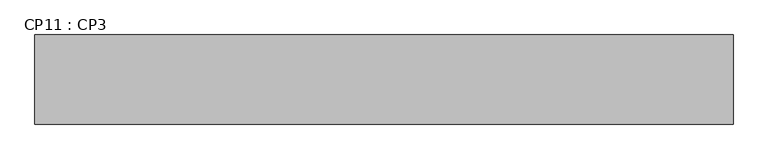
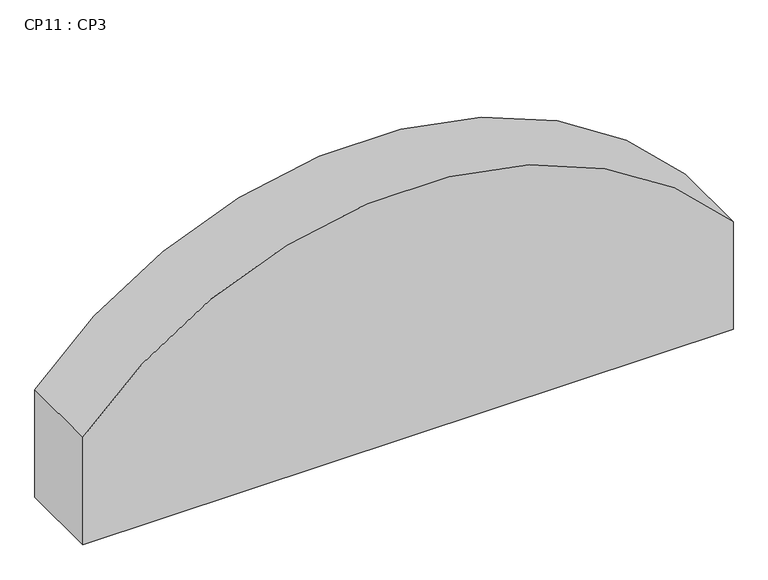
"""IFC4 building model written with IfcOpenShell, lengths in millimetres: beam geometry, CP11 : CP3."""

import ifcopenshell
import ifcopenshell.guid

model = None  # the IFC model being written
_history = None  # IfcOwnerHistory: only IFC2X3 demands one
_inside = {}  # id of a spatial element -> (the spatial element, [elements in it])
_under = {}  # id of a project, library or spatial element -> (it, [spatial elements below it])
_declared = {}  # id of a project -> (the project, [libraries it declares])
_typed = {}  # id of a type object -> (the type object, [elements of that type])
_made_of = {}  # id of a material, layer set ... -> (it, [elements and type objects made of it])


def new_model(schema):
    """Start an empty IFC model of exactly this schema.

    Asked for "IFC4X3", IfcOpenShell would pick the latest addendum, in which some entities
    have other attributes; the version numbers below select the first issue.
    IFC2X3 requires an IfcOwnerHistory on every rooted entity: one is made here for all.
    """
    global model, _history
    if schema == "IFC4X3":
        model = ifcopenshell.file(schema_version=(4, 3, 0, 0))
    else:
        model = ifcopenshell.file(schema=schema)
    _inside.clear()
    _under.clear()
    _declared.clear()
    _typed.clear()
    _made_of.clear()
    _history = None
    if model.schema == "IFC2X3":
        org = make("IfcOrganization", Name="unknown")
        user = make(
            "IfcPersonAndOrganization",
            ThePerson=make("IfcPerson", FamilyName="unknown"),
            TheOrganization=org,
        )
        app = make(
            "IfcApplication",
            ApplicationDeveloper=org,
            Version="unknown",
            ApplicationFullName="unknown",
            ApplicationIdentifier="unknown",
        )
        _history = make(
            "IfcOwnerHistory",
            OwningUser=user,
            OwningApplication=app,
            ChangeAction="ADDED",
            CreationDate=0,
        )
    return model


def make(cls, **values):
    """One entity of the class cls with the attributes given. An attribute that is None is left unset."""
    return model.create_entity(
        cls, **{name: value for name, value in values.items() if value is not None}
    )


def rooted(cls, **values):
    """An entity with a GlobalId (a new one), such as an element, a storey or a relation."""
    return make(cls, GlobalId=ifcopenshell.guid.new(), OwnerHistory=_history, **values)


def si_unit(unit_type, name, prefix=None):
    """IfcSIUnit, for example si_unit("LENGTHUNIT", "METRE", prefix="MILLI")."""
    return make("IfcSIUnit", UnitType=unit_type, Prefix=prefix, Name=name)


def assignment(units):
    """IfcUnitAssignment: the units of a project."""
    return None if units is None else make("IfcUnitAssignment", Units=units)


def point(xyz):
    """IfcCartesianPoint."""
    return None if xyz is None else make("IfcCartesianPoint", Coordinates=xyz)


def direction(xyz):
    """IfcDirection."""
    return None if xyz is None else make("IfcDirection", DirectionRatios=xyz)


def frame(location, z_axis=None, x_axis=None):
    """IfcAxis2Placement3D, a coordinate frame: its origin and axes. An axis left out is left unset."""
    return make(
        "IfcAxis2Placement3D",
        Location=point(location),
        Axis=direction(z_axis),
        RefDirection=direction(x_axis),
    )


def origin():
    """The frame at (0, 0, 0) with its axes left unset."""
    return frame((0.0, 0.0, 0.0))


def place(relative_to, where):
    """IfcLocalPlacement: puts the frame where relative to a parent placement (None: the world)."""
    return make(
        "IfcLocalPlacement", PlacementRelTo=relative_to, RelativePlacement=where
    )


def context(
    kind, dimensions, precision=None, world=None, true_north=None, identifier=None
):
    """IfcGeometricRepresentationContext, for example the 3D "Model" context."""
    return make(
        "IfcGeometricRepresentationContext",
        ContextIdentifier=identifier,
        ContextType=kind,
        CoordinateSpaceDimension=dimensions,
        Precision=precision,
        WorldCoordinateSystem=world,
        TrueNorth=true_north,
    )


def project(units=None, contexts=None):
    """IfcProject with its units and contexts."""
    return rooted(
        "IfcProject",
        Name="project",
        RepresentationContexts=contexts,
        UnitsInContext=assignment(units),
    )


def spatial(cls, under=None, at=None, **own):
    """A site, building, storey or space (cls), placed at a placement, below another one or the project."""
    s = rooted(cls, ObjectPlacement=at, **own)
    if under is not None:
        _under.setdefault(under.id(), (under, []))[1].append(s)
    return s


def circle_curve(where, radius):
    """IfcCircle in the frame where."""
    return make("IfcCircle", Position=where, Radius=radius)


def shape(context_of_items, identifier, shape_type, items):
    """IfcShapeRepresentation: the items that make up one representation, for example the "Body"."""
    return make(
        "IfcShapeRepresentation",
        ContextOfItems=context_of_items,
        RepresentationIdentifier=identifier,
        RepresentationType=shape_type,
        Items=items,
    )


def source(mapping_origin, context_of_items, identifier, shape_type, items):
    """IfcRepresentationMap: a shape defined once, which mapped items show again and again."""
    return make(
        "IfcRepresentationMap",
        MappingOrigin=mapping_origin,
        MappedRepresentation=shape(context_of_items, identifier, shape_type, items),
    )


def transform(
    local_origin,
    x_axis=None,
    y_axis=None,
    z_axis=None,
    scale=None,
    scale2=None,
    scale3=None,
    uniform=True,
):
    """IfcCartesianTransformationOperator3D, or its non-uniform kind. x_axis, y_axis, z_axis: its Axis1, 2, 3."""
    if uniform:
        return make(
            "IfcCartesianTransformationOperator3D",
            Axis1=direction(x_axis),
            Axis2=direction(y_axis),
            LocalOrigin=point(local_origin),
            Scale=scale,
            Axis3=direction(z_axis),
        )
    return make(
        "IfcCartesianTransformationOperator3DnonUniform",
        Axis1=direction(x_axis),
        Axis2=direction(y_axis),
        LocalOrigin=point(local_origin),
        Scale=scale,
        Axis3=direction(z_axis),
        Scale2=scale2,
        Scale3=scale3,
    )


def mapped(mapping_source, mapping_target):
    """IfcMappedItem: shows the shape of a source again, moved by a transform."""
    return make(
        "IfcMappedItem", MappingSource=mapping_source, MappingTarget=mapping_target
    )


def made_of(thing, what):
    """Note that an element or type object is made of a material, layer set ...; save() writes the relation."""
    if what is not None:
        _made_of.setdefault(what.id(), (what, []))[1].append(thing)
    return thing


def element(
    cls,
    number,
    at=None,
    inside=None,
    cuts=None,
    type_object=None,
    material=None,
    context=None,
    identifier="Body",
    shape_type=None,
    held_by="IfcProductDefinitionShape",
    body=None,
    shapes=None,
    **own,
):
    """One element of the class cls, such as IfcWall. Its Tag is "e" and its number.

    at: its placement. inside: the storey or other place that contains it. cuts: it is an
    opening in that element (IfcRelVoidsElement). A single representation is given by context,
    identifier, shape_type and body (its items); several are given by shapes. held_by: the class
    of the entity that holds the representations. save() writes the other relations.
    """
    e = rooted(cls, Tag="e%d" % number, ObjectPlacement=at, **own)
    if body is not None:
        shapes = [shape(context, identifier, shape_type, body)]
    if shapes is not None:
        e.Representation = make(held_by, Representations=shapes)
    if inside is not None:
        _inside.setdefault(inside.id(), (inside, []))[1].append(e)
    if cuts is not None:
        rooted(
            "IfcRelVoidsElement", RelatingBuildingElement=cuts, RelatedOpeningElement=e
        )
    if type_object is not None:
        _typed.setdefault(type_object.id(), (type_object, []))[1].append(e)
    return made_of(e, material)


def aggregate(whole, parts):
    """IfcRelAggregates: a whole, such as a stair, and the parts it consists of."""
    return rooted("IfcRelAggregates", RelatingObject=whole, RelatedObjects=parts)


def save(model, path):
    """Write the relations noted so far, then the file.

    IfcRelAggregates (storeys below a building ...), IfcRelContainedInSpatialStructure (elements
    in a storey), IfcRelDefinesByType, IfcRelAssociatesMaterial and IfcRelDeclares: one each for
    every whole, place, type object, material and project.
    """
    for whole, parts in _under.values():
        aggregate(whole, parts)
    for where, things in _inside.values():
        rooted(
            "IfcRelContainedInSpatialStructure",
            RelatedElements=things,
            RelatingStructure=where,
        )
    for kind, things in _typed.values():
        rooted("IfcRelDefinesByType", RelatedObjects=things, RelatingType=kind)
    for what, things in _made_of.values():
        rooted("IfcRelAssociatesMaterial", RelatedObjects=things, RelatingMaterial=what)
    for by, libraries in _declared.values():
        rooted("IfcRelDeclares", RelatingContext=by, RelatedDefinitions=libraries)
    model.write(path)


def plane_surface(at):
    """IfcPlane: the flat surface through the origin of the frame at, square to its z axis."""
    return make("IfcPlane", Position=at)


def cylinder_surface(at, radius):
    """IfcCylindricalSurface: all points at the distance radius from the z axis of the frame at."""
    return make("IfcCylindricalSurface", Position=at, Radius=radius)


def advanced_brep(points, edges, surfaces, faces):
    """IfcAdvancedBrep: a solid bounded by faces that lie on surfaces and meet in shared edges.

    An edge is (start, end): straight between two places in points (the first is 0);
    or (start, end, curve); or (start, end, curve, False) where it runs against its curve.
    A face is (place in surfaces, loops), or (place, loops, False) where it looks against
    its surface's normal. A loop lists edges by number (the first is 1), with a minus sign
    where the edge is run from its end to its start. The first loop is the outer one.
    """
    corners = [point(p) for p in points]
    vertices = [make("IfcVertexPoint", VertexGeometry=c) for c in corners]
    made = []
    for start, end, *more in edges:
        made.append(
            make(
                "IfcEdgeCurve",
                EdgeStart=vertices[start],
                EdgeEnd=vertices[end],
                EdgeGeometry=more[0] if more else make("IfcPolyline", Points=[corners[start], corners[end]]),
                SameSense=more[1] if len(more) > 1 else True,
            )
        )
    hull = []
    for where, loops, *sense in faces:
        bounds = []
        for j, loop in enumerate(loops):
            ring = [make("IfcOrientedEdge", EdgeElement=made[abs(k) - 1], Orientation=k > 0) for k in loop]
            bounds.append(
                make(
                    "IfcFaceOuterBound" if j == 0 else "IfcFaceBound",
                    Bound=make("IfcEdgeLoop", EdgeList=ring),
                    Orientation=True,
                )
            )
        hull.append(make("IfcAdvancedFace", Bounds=bounds, FaceSurface=surfaces[where], SameSense=sense[0] if sense else True))
    return make("IfcAdvancedBrep", Outer=make("IfcClosedShell", CfsFaces=hull))


def cp11_cp3_567e5ed8(model_context):
    return source(origin(), model_context, "Body", "AdvancedBrep", [
        advanced_brep(
        [(35483.2245514, 499.6999991, 14620.0), (40183.2245513, 499.6999991, 14620.0), (40183.22455, 499.6999991, 13800.0), (35483.2245494, 499.6999991, 13800.0), (40183.2245513, -100.2551788, 14620.0), (35483.2245514, -100.2551788, 14620.0), (35483.2245494, -100.2551788, 13800.0), (40183.22455, -100.2551788, 13800.0)],
        [
            (0, 1, circle_curve(frame((37833.2245514, 499.6999991, 12603.2870371), z_axis=(0.0, 1.0, 0.0), x_axis=(0.0, 0.0, -1.0)), 3096.7129629)),
            (1, 2),
            (2, 3),
            (3, 0),
            (4, 5, circle_curve(frame((37833.2245514, -100.2551788, 12603.2870371), z_axis=(0.0, -1.0, 0.0), x_axis=(0.0, 0.0, -1.0)), 3096.7129629)),
            (5, 6),
            (6, 7),
            (7, 4),
            (6, 3),
            (2, 7),
            (0, 5),
            (4, 1),
        ],
        [
            plane_surface(frame((35333.2245515, 499.6999991, 13800.0), z_axis=(0.0, 1.0, 0.0), x_axis=(0.0, 0.0, 1.0))),
            plane_surface(frame((35333.2245515, -100.2551788, 13800.0), z_axis=(0.0, -1.0, 0.0), x_axis=(0.0, 0.0, -1.0))),
            plane_surface(frame((40333.2245515, 499.6999991, 13800.0), z_axis=(0.0, 0.0, -1.0), x_axis=(0.0, -1.0, 0.0))),
            cylinder_surface(frame((37833.2245514, 20099.7448193, 12603.2870371), z_axis=(0.0, 1.0, 0.0), x_axis=(0.0, 0.0, -1.0)), 3096.7129629),
            plane_surface(frame((35483.2245494, 18587.0448193, 14620.0), z_axis=(-1.0, 0.0, 0.0), x_axis=(0.0, -1.0, 0.0))),
            plane_surface(frame((40183.22455, 18587.0448193, 13800.0), z_axis=(1.0, 0.0, 0.0), x_axis=(0.0, -1.0, 0.0))),
        ],
        [
            (0, [[1, 2, 3, 4]]),
            (1, [[5, 6, 7, 8]]),
            (2, [[9, -3, 10, -7]]),
            (3, [[-1, 11, -5, 12]]),
            (4, [[-4, -9, -6, -11]]),
            (5, [[-2, -12, -8, -10]]),
        ],
    ),
    ])


if __name__ == "__main__":
    model = new_model("IFC4")
    model_context = context("Model", 3, world=origin())
    ifc_project = project(units=[si_unit("LENGTHUNIT", "METRE", prefix="MILLI")], contexts=[model_context])
    site = spatial("IfcSite", under=ifc_project)
    building = spatial("IfcBuilding", under=site)
    placement = place(None, origin())
    cp11_cp3_shape = cp11_cp3_567e5ed8(model_context)
    element("IfcBeam", 1, ObjectType="CP11 : CP3", at=placement, inside=building, context=model_context, shape_type="MappedRepresentation", body=[
        mapped(cp11_cp3_shape, transform((0.0, 0.0, 0.0), x_axis=(1.0, 0.0, 0.0), y_axis=(0.0, 1.0, 0.0), z_axis=(0.0, 0.0, 1.0))),
    ])
    save(model, "model.ifc")
